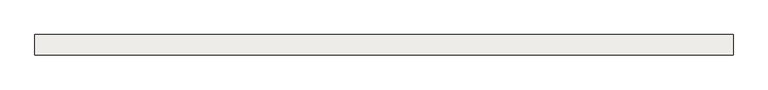
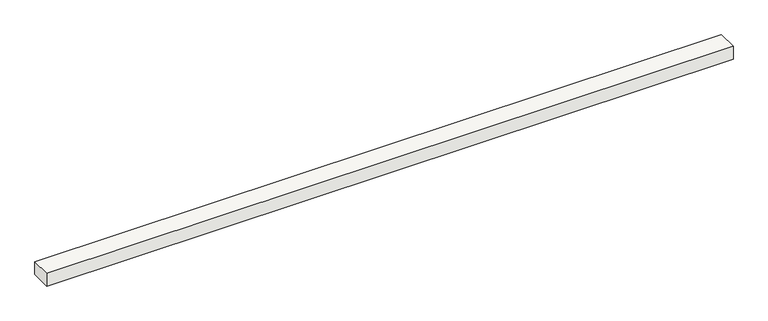
"""IFC4 building model written with IfcOpenShell, lengths in millimetres: slab geometry, Ditch 2 : Ditch 2."""

from ifc_helpers import new_model, si_unit, frame, origin, place, context, project, spatial, polyline, outline, extrude, source, transform, mapped, element, save


def slab_e6aba4ee(model_context):
    return source(origin(), model_context, "Body", "SweptSolid", [
        extrude(outline(polyline([(100.0, 18194.5382614), (100.0, 18494.5382614), (10325.0, 18494.5382614), (10325.0, 18194.5382614), (100.0, 18194.5382614)])), frame((0.0, 0.0, -500.0), z_axis=(0.0, 0.0, 1.0), x_axis=(1.0, 0.0, 0.0)), (0.0, 0.0, 1.0), 200.0),
    ])


if __name__ == "__main__":
    model = new_model("IFC4")
    model_context = context("Model", 3, world=origin())
    ifc_project = project(units=[si_unit("LENGTHUNIT", "METRE", prefix="MILLI")], contexts=[model_context])
    site = spatial("IfcSite", under=ifc_project)
    building = spatial("IfcBuilding", under=site)
    placement = place(None, origin())
    slab_shape = slab_e6aba4ee(model_context)
    element("IfcSlab", 1, ObjectType="Ditch 2 : Ditch 2", at=placement, inside=building, context=model_context, shape_type="MappedRepresentation", body=[
        mapped(slab_shape, transform((0.0, 0.0, 0.0), x_axis=(1.0, 0.0, 0.0), y_axis=(0.0, 1.0, 0.0), z_axis=(0.0, 0.0, 1.0))),
    ])
    save(model, "model.ifc")

# Revit data of these elements
# Element 1 (IfcSlab, "Ditch 2 : Ditch 2")
#   Materials on its faces: "A03AC032-00007_Structural Concrete_Type1_25MPa-30Mpa"
# Materials
#   "A03AC032-00007_Structural Concrete_Type1_25MPa-30Mpa": class "Concrete", colour RGB 176 176 176, transparency 0, Keynote = "09910.A1", Description = "Reinf. Conc.", W00) Work Master Code = "A03AC032-00007", W01) Work Master_Lv1 = "Concrete Work", W02) Work Master_Lv2 = "Substructure Work", W03) Work Master_Spec.1 = "Structural Concrete", W04) Work Master_Spec.2 = "Cement Type-1", W05) Work Master_Spec.3 = "25MPa < F'c (Cylinder Strength) ≤ 30MPa", Cost = 0
